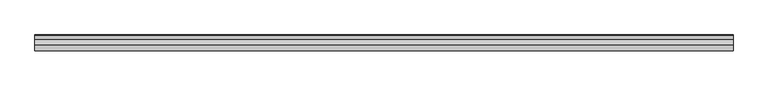
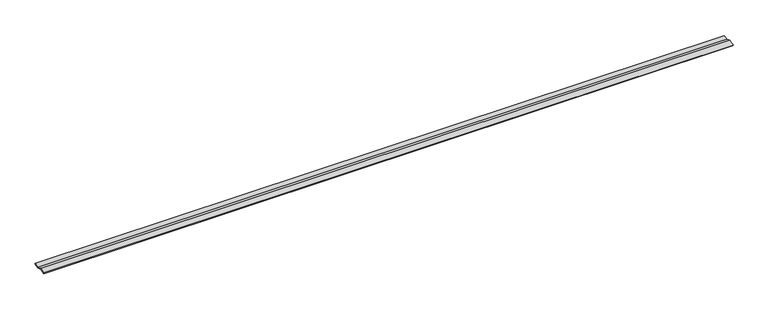
"""IFC4 building model written with IfcOpenShell, lengths in millimetres: proxy geometry, Gutter @ Roof004 : Gutter @ Roof004."""

import ifcopenshell
import ifcopenshell.guid

model = None  # the IFC model being written
_history = None  # IfcOwnerHistory: only IFC2X3 demands one
_inside = {}  # id of a spatial element -> (the spatial element, [elements in it])
_under = {}  # id of a project, library or spatial element -> (it, [spatial elements below it])
_declared = {}  # id of a project -> (the project, [libraries it declares])
_typed = {}  # id of a type object -> (the type object, [elements of that type])
_made_of = {}  # id of a material, layer set ... -> (it, [elements and type objects made of it])


def new_model(schema):
    """Start an empty IFC model of exactly this schema.

    Asked for "IFC4X3", IfcOpenShell would pick the latest addendum, in which some entities
    have other attributes; the version numbers below select the first issue.
    IFC2X3 requires an IfcOwnerHistory on every rooted entity: one is made here for all.
    """
    global model, _history
    if schema == "IFC4X3":
        model = ifcopenshell.file(schema_version=(4, 3, 0, 0))
    else:
        model = ifcopenshell.file(schema=schema)
    _inside.clear()
    _under.clear()
    _declared.clear()
    _typed.clear()
    _made_of.clear()
    _history = None
    if model.schema == "IFC2X3":
        org = make("IfcOrganization", Name="unknown")
        user = make(
            "IfcPersonAndOrganization",
            ThePerson=make("IfcPerson", FamilyName="unknown"),
            TheOrganization=org,
        )
        app = make(
            "IfcApplication",
            ApplicationDeveloper=org,
            Version="unknown",
            ApplicationFullName="unknown",
            ApplicationIdentifier="unknown",
        )
        _history = make(
            "IfcOwnerHistory",
            OwningUser=user,
            OwningApplication=app,
            ChangeAction="ADDED",
            CreationDate=0,
        )
    return model


def make(cls, **values):
    """One entity of the class cls with the attributes given. An attribute that is None is left unset."""
    return model.create_entity(
        cls, **{name: value for name, value in values.items() if value is not None}
    )


def rooted(cls, **values):
    """An entity with a GlobalId (a new one), such as an element, a storey or a relation."""
    return make(cls, GlobalId=ifcopenshell.guid.new(), OwnerHistory=_history, **values)


def si_unit(unit_type, name, prefix=None):
    """IfcSIUnit, for example si_unit("LENGTHUNIT", "METRE", prefix="MILLI")."""
    return make("IfcSIUnit", UnitType=unit_type, Prefix=prefix, Name=name)


def assignment(units):
    """IfcUnitAssignment: the units of a project."""
    return None if units is None else make("IfcUnitAssignment", Units=units)


def point(xyz):
    """IfcCartesianPoint."""
    return None if xyz is None else make("IfcCartesianPoint", Coordinates=xyz)


def direction(xyz):
    """IfcDirection."""
    return None if xyz is None else make("IfcDirection", DirectionRatios=xyz)


def frame(location, z_axis=None, x_axis=None):
    """IfcAxis2Placement3D, a coordinate frame: its origin and axes. An axis left out is left unset."""
    return make(
        "IfcAxis2Placement3D",
        Location=point(location),
        Axis=direction(z_axis),
        RefDirection=direction(x_axis),
    )


def origin():
    """The frame at (0, 0, 0) with its axes left unset."""
    return frame((0.0, 0.0, 0.0))


def place(relative_to, where):
    """IfcLocalPlacement: puts the frame where relative to a parent placement (None: the world)."""
    return make(
        "IfcLocalPlacement", PlacementRelTo=relative_to, RelativePlacement=where
    )


def context(
    kind, dimensions, precision=None, world=None, true_north=None, identifier=None
):
    """IfcGeometricRepresentationContext, for example the 3D "Model" context."""
    return make(
        "IfcGeometricRepresentationContext",
        ContextIdentifier=identifier,
        ContextType=kind,
        CoordinateSpaceDimension=dimensions,
        Precision=precision,
        WorldCoordinateSystem=world,
        TrueNorth=true_north,
    )


def project(units=None, contexts=None):
    """IfcProject with its units and contexts."""
    return rooted(
        "IfcProject",
        Name="project",
        RepresentationContexts=contexts,
        UnitsInContext=assignment(units),
    )


def spatial(cls, under=None, at=None, **own):
    """A site, building, storey or space (cls), placed at a placement, below another one or the project."""
    s = rooted(cls, ObjectPlacement=at, **own)
    if under is not None:
        _under.setdefault(under.id(), (under, []))[1].append(s)
    return s


def polyline(points):
    """IfcPolyline through the points."""
    return make("IfcPolyline", Points=[point(p) for p in points])


def outline(outer, holes=None, kind="AREA"):
    """IfcArbitraryClosedProfileDef: a profile drawn as a closed curve; with holes, ...WithVoids."""
    if holes is None:
        return make("IfcArbitraryClosedProfileDef", ProfileType=kind, OuterCurve=outer)
    return make(
        "IfcArbitraryProfileDefWithVoids",
        ProfileType=kind,
        OuterCurve=outer,
        InnerCurves=holes,
    )


def extrude(swept, where, along, depth):
    """IfcExtrudedAreaSolid: the profile swept, set in the frame where, extruded along a direction by depth."""
    return make(
        "IfcExtrudedAreaSolid",
        SweptArea=swept,
        Position=where,
        ExtrudedDirection=direction(along),
        Depth=depth,
    )


def shape(context_of_items, identifier, shape_type, items):
    """IfcShapeRepresentation: the items that make up one representation, for example the "Body"."""
    return make(
        "IfcShapeRepresentation",
        ContextOfItems=context_of_items,
        RepresentationIdentifier=identifier,
        RepresentationType=shape_type,
        Items=items,
    )


def source(mapping_origin, context_of_items, identifier, shape_type, items):
    """IfcRepresentationMap: a shape defined once, which mapped items show again and again."""
    return make(
        "IfcRepresentationMap",
        MappingOrigin=mapping_origin,
        MappedRepresentation=shape(context_of_items, identifier, shape_type, items),
    )


def transform(
    local_origin,
    x_axis=None,
    y_axis=None,
    z_axis=None,
    scale=None,
    scale2=None,
    scale3=None,
    uniform=True,
):
    """IfcCartesianTransformationOperator3D, or its non-uniform kind. x_axis, y_axis, z_axis: its Axis1, 2, 3."""
    if uniform:
        return make(
            "IfcCartesianTransformationOperator3D",
            Axis1=direction(x_axis),
            Axis2=direction(y_axis),
            LocalOrigin=point(local_origin),
            Scale=scale,
            Axis3=direction(z_axis),
        )
    return make(
        "IfcCartesianTransformationOperator3DnonUniform",
        Axis1=direction(x_axis),
        Axis2=direction(y_axis),
        LocalOrigin=point(local_origin),
        Scale=scale,
        Axis3=direction(z_axis),
        Scale2=scale2,
        Scale3=scale3,
    )


def mapped(mapping_source, mapping_target):
    """IfcMappedItem: shows the shape of a source again, moved by a transform."""
    return make(
        "IfcMappedItem", MappingSource=mapping_source, MappingTarget=mapping_target
    )


def made_of(thing, what):
    """Note that an element or type object is made of a material, layer set ...; save() writes the relation."""
    if what is not None:
        _made_of.setdefault(what.id(), (what, []))[1].append(thing)
    return thing


def element(
    cls,
    number,
    at=None,
    inside=None,
    cuts=None,
    type_object=None,
    material=None,
    context=None,
    identifier="Body",
    shape_type=None,
    held_by="IfcProductDefinitionShape",
    body=None,
    shapes=None,
    **own,
):
    """One element of the class cls, such as IfcWall. Its Tag is "e" and its number.

    at: its placement. inside: the storey or other place that contains it. cuts: it is an
    opening in that element (IfcRelVoidsElement). A single representation is given by context,
    identifier, shape_type and body (its items); several are given by shapes. held_by: the class
    of the entity that holds the representations. save() writes the other relations.
    """
    e = rooted(cls, Tag="e%d" % number, ObjectPlacement=at, **own)
    if body is not None:
        shapes = [shape(context, identifier, shape_type, body)]
    if shapes is not None:
        e.Representation = make(held_by, Representations=shapes)
    if inside is not None:
        _inside.setdefault(inside.id(), (inside, []))[1].append(e)
    if cuts is not None:
        rooted(
            "IfcRelVoidsElement", RelatingBuildingElement=cuts, RelatedOpeningElement=e
        )
    if type_object is not None:
        _typed.setdefault(type_object.id(), (type_object, []))[1].append(e)
    return made_of(e, material)


def aggregate(whole, parts):
    """IfcRelAggregates: a whole, such as a stair, and the parts it consists of."""
    return rooted("IfcRelAggregates", RelatingObject=whole, RelatedObjects=parts)


def save(model, path):
    """Write the relations noted so far, then the file.

    IfcRelAggregates (storeys below a building ...), IfcRelContainedInSpatialStructure (elements
    in a storey), IfcRelDefinesByType, IfcRelAssociatesMaterial and IfcRelDeclares: one each for
    every whole, place, type object, material and project.
    """
    for whole, parts in _under.values():
        aggregate(whole, parts)
    for where, things in _inside.values():
        rooted(
            "IfcRelContainedInSpatialStructure",
            RelatedElements=things,
            RelatingStructure=where,
        )
    for kind, things in _typed.values():
        rooted("IfcRelDefinesByType", RelatedObjects=things, RelatingType=kind)
    for what, things in _made_of.values():
        rooted("IfcRelAssociatesMaterial", RelatedObjects=things, RelatingMaterial=what)
    for by, libraries in _declared.values():
        rooted("IfcRelDeclares", RelatingContext=by, RelatedDefinitions=libraries)
    model.write(path)


def generic_models_2a12b37d(model_context):
    return source(origin(), model_context, "Body", "SweptSolid", [
        extrude(outline(polyline([(-5227.7746422, 42846.6894729), (-5213.6083006, 42841.7188154), (-5200.2540881, 42845.1047805), (-5199.629824, 42842.6426891), (-5213.726504, 42839.0684711), (-5227.8868147, 42844.0370125), (-5243.936465, 42839.8887832), (-5244.5720722, 42842.3479707), (-5227.7746422, 42846.6894729)])), frame((12382.7678845, 0.0, 0.0), z_axis=(1.0, 0.0, 0.0), x_axis=(0.0, 1.0, 0.0)), (0.0, 0.0, 1.0), 2000.25),
    ])


if __name__ == "__main__":
    model = new_model("IFC4")
    model_context = context("Model", 3, world=origin())
    ifc_project = project(units=[si_unit("LENGTHUNIT", "METRE", prefix="MILLI")], contexts=[model_context])
    site = spatial("IfcSite", under=ifc_project)
    building = spatial("IfcBuilding", under=site)
    placement = place(None, origin())
    generic_models_shape = generic_models_2a12b37d(model_context)
    element("IfcBuildingElementProxy", 1, Name="Gutter @ Roof004 : Gutter @ Roof004", ObjectType="Gutter @ Roof004 : Gutter @ Roof004", at=placement, inside=building, context=model_context, shape_type="MappedRepresentation", body=[
        mapped(generic_models_shape, transform((0.0, 0.0, 0.0), x_axis=(1.0, 0.0, 0.0), y_axis=(0.0, 1.0, 0.0), z_axis=(0.0, 0.0, 1.0))),
    ])
    save(model, "model.ifc")

# Revit data of these elements
# Type "Gutter @ Roof004 : Gutter @ Roof004"
#   NameOverride = "Gutter @ Roof004"
# Element 1 (IfcBuildingElementProxy, "Gutter @ Roof004 : Gutter @ Roof004")
#   Materials on its faces: "CONT. SEAMLESS 16 GA COPPER BRAKE METAL GUTTER"
# Materials
#   "CONT. SEAMLESS 16 GA COPPER BRAKE METAL GUTTER": class "Unassigned", colour RGB 128 128 128, transparency 0
